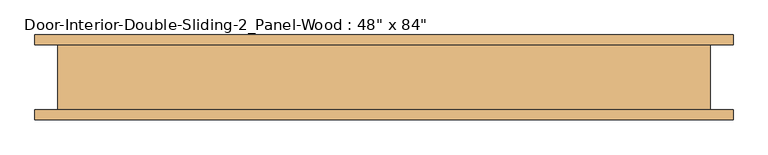
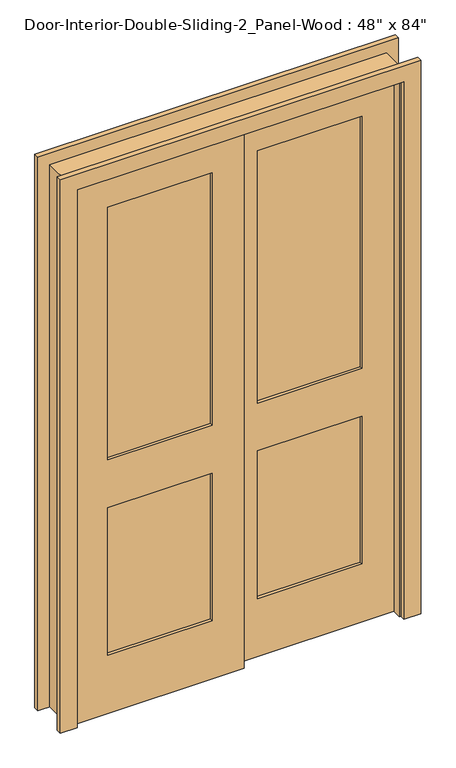
"""IFC4 building model written with IfcOpenShell, lengths in millimetres: door geometry."""

import ifcopenshell
import ifcopenshell.guid

model = None  # the IFC model being written
_history = None  # IfcOwnerHistory: only IFC2X3 demands one
_inside = {}  # id of a spatial element -> (the spatial element, [elements in it])
_under = {}  # id of a project, library or spatial element -> (it, [spatial elements below it])
_declared = {}  # id of a project -> (the project, [libraries it declares])
_typed = {}  # id of a type object -> (the type object, [elements of that type])
_made_of = {}  # id of a material, layer set ... -> (it, [elements and type objects made of it])


def new_model(schema):
    """Start an empty IFC model of exactly this schema.

    Asked for "IFC4X3", IfcOpenShell would pick the latest addendum, in which some entities
    have other attributes; the version numbers below select the first issue.
    IFC2X3 requires an IfcOwnerHistory on every rooted entity: one is made here for all.
    """
    global model, _history
    if schema == "IFC4X3":
        model = ifcopenshell.file(schema_version=(4, 3, 0, 0))
    else:
        model = ifcopenshell.file(schema=schema)
    _inside.clear()
    _under.clear()
    _declared.clear()
    _typed.clear()
    _made_of.clear()
    _history = None
    if model.schema == "IFC2X3":
        org = make("IfcOrganization", Name="unknown")
        user = make(
            "IfcPersonAndOrganization",
            ThePerson=make("IfcPerson", FamilyName="unknown"),
            TheOrganization=org,
        )
        app = make(
            "IfcApplication",
            ApplicationDeveloper=org,
            Version="unknown",
            ApplicationFullName="unknown",
            ApplicationIdentifier="unknown",
        )
        _history = make(
            "IfcOwnerHistory",
            OwningUser=user,
            OwningApplication=app,
            ChangeAction="ADDED",
            CreationDate=0,
        )
    return model


def make(cls, **values):
    """One entity of the class cls with the attributes given. An attribute that is None is left unset."""
    return model.create_entity(
        cls, **{name: value for name, value in values.items() if value is not None}
    )


def rooted(cls, **values):
    """An entity with a GlobalId (a new one), such as an element, a storey or a relation."""
    return make(cls, GlobalId=ifcopenshell.guid.new(), OwnerHistory=_history, **values)


def si_unit(unit_type, name, prefix=None):
    """IfcSIUnit, for example si_unit("LENGTHUNIT", "METRE", prefix="MILLI")."""
    return make("IfcSIUnit", UnitType=unit_type, Prefix=prefix, Name=name)


def assignment(units):
    """IfcUnitAssignment: the units of a project."""
    return None if units is None else make("IfcUnitAssignment", Units=units)


def point(xyz):
    """IfcCartesianPoint."""
    return None if xyz is None else make("IfcCartesianPoint", Coordinates=xyz)


def direction(xyz):
    """IfcDirection."""
    return None if xyz is None else make("IfcDirection", DirectionRatios=xyz)


def frame(location, z_axis=None, x_axis=None):
    """IfcAxis2Placement3D, a coordinate frame: its origin and axes. An axis left out is left unset."""
    return make(
        "IfcAxis2Placement3D",
        Location=point(location),
        Axis=direction(z_axis),
        RefDirection=direction(x_axis),
    )


def origin():
    """The frame at (0, 0, 0) with its axes left unset."""
    return frame((0.0, 0.0, 0.0))


def place(relative_to, where):
    """IfcLocalPlacement: puts the frame where relative to a parent placement (None: the world)."""
    return make(
        "IfcLocalPlacement", PlacementRelTo=relative_to, RelativePlacement=where
    )


def context(
    kind, dimensions, precision=None, world=None, true_north=None, identifier=None
):
    """IfcGeometricRepresentationContext, for example the 3D "Model" context."""
    return make(
        "IfcGeometricRepresentationContext",
        ContextIdentifier=identifier,
        ContextType=kind,
        CoordinateSpaceDimension=dimensions,
        Precision=precision,
        WorldCoordinateSystem=world,
        TrueNorth=true_north,
    )


def project(units=None, contexts=None):
    """IfcProject with its units and contexts."""
    return rooted(
        "IfcProject",
        Name="project",
        RepresentationContexts=contexts,
        UnitsInContext=assignment(units),
    )


def spatial(cls, under=None, at=None, **own):
    """A site, building, storey or space (cls), placed at a placement, below another one or the project."""
    s = rooted(cls, ObjectPlacement=at, **own)
    if under is not None:
        _under.setdefault(under.id(), (under, []))[1].append(s)
    return s


def polyline(points):
    """IfcPolyline through the points."""
    return make("IfcPolyline", Points=[point(p) for p in points])


def outline(outer, holes=None, kind="AREA"):
    """IfcArbitraryClosedProfileDef: a profile drawn as a closed curve; with holes, ...WithVoids."""
    if holes is None:
        return make("IfcArbitraryClosedProfileDef", ProfileType=kind, OuterCurve=outer)
    return make(
        "IfcArbitraryProfileDefWithVoids",
        ProfileType=kind,
        OuterCurve=outer,
        InnerCurves=holes,
    )


def extrude(swept, where, along, depth):
    """IfcExtrudedAreaSolid: the profile swept, set in the frame where, extruded along a direction by depth."""
    return make(
        "IfcExtrudedAreaSolid",
        SweptArea=swept,
        Position=where,
        ExtrudedDirection=direction(along),
        Depth=depth,
    )


def shape(context_of_items, identifier, shape_type, items):
    """IfcShapeRepresentation: the items that make up one representation, for example the "Body"."""
    return make(
        "IfcShapeRepresentation",
        ContextOfItems=context_of_items,
        RepresentationIdentifier=identifier,
        RepresentationType=shape_type,
        Items=items,
    )


def source(mapping_origin, context_of_items, identifier, shape_type, items):
    """IfcRepresentationMap: a shape defined once, which mapped items show again and again."""
    return make(
        "IfcRepresentationMap",
        MappingOrigin=mapping_origin,
        MappedRepresentation=shape(context_of_items, identifier, shape_type, items),
    )


def transform(
    local_origin,
    x_axis=None,
    y_axis=None,
    z_axis=None,
    scale=None,
    scale2=None,
    scale3=None,
    uniform=True,
):
    """IfcCartesianTransformationOperator3D, or its non-uniform kind. x_axis, y_axis, z_axis: its Axis1, 2, 3."""
    if uniform:
        return make(
            "IfcCartesianTransformationOperator3D",
            Axis1=direction(x_axis),
            Axis2=direction(y_axis),
            LocalOrigin=point(local_origin),
            Scale=scale,
            Axis3=direction(z_axis),
        )
    return make(
        "IfcCartesianTransformationOperator3DnonUniform",
        Axis1=direction(x_axis),
        Axis2=direction(y_axis),
        LocalOrigin=point(local_origin),
        Scale=scale,
        Axis3=direction(z_axis),
        Scale2=scale2,
        Scale3=scale3,
    )


def mapped(mapping_source, mapping_target):
    """IfcMappedItem: shows the shape of a source again, moved by a transform."""
    return make(
        "IfcMappedItem", MappingSource=mapping_source, MappingTarget=mapping_target
    )


def made_of(thing, what):
    """Note that an element or type object is made of a material, layer set ...; save() writes the relation."""
    if what is not None:
        _made_of.setdefault(what.id(), (what, []))[1].append(thing)
    return thing


def element(
    cls,
    number,
    at=None,
    inside=None,
    cuts=None,
    type_object=None,
    material=None,
    context=None,
    identifier="Body",
    shape_type=None,
    held_by="IfcProductDefinitionShape",
    body=None,
    shapes=None,
    **own,
):
    """One element of the class cls, such as IfcWall. Its Tag is "e" and its number.

    at: its placement. inside: the storey or other place that contains it. cuts: it is an
    opening in that element (IfcRelVoidsElement). A single representation is given by context,
    identifier, shape_type and body (its items); several are given by shapes. held_by: the class
    of the entity that holds the representations. save() writes the other relations.
    """
    e = rooted(cls, Tag="e%d" % number, ObjectPlacement=at, **own)
    if body is not None:
        shapes = [shape(context, identifier, shape_type, body)]
    if shapes is not None:
        e.Representation = make(held_by, Representations=shapes)
    if inside is not None:
        _inside.setdefault(inside.id(), (inside, []))[1].append(e)
    if cuts is not None:
        rooted(
            "IfcRelVoidsElement", RelatingBuildingElement=cuts, RelatedOpeningElement=e
        )
    if type_object is not None:
        _typed.setdefault(type_object.id(), (type_object, []))[1].append(e)
    return made_of(e, material)


def aggregate(whole, parts):
    """IfcRelAggregates: a whole, such as a stair, and the parts it consists of."""
    return rooted("IfcRelAggregates", RelatingObject=whole, RelatedObjects=parts)


def save(model, path):
    """Write the relations noted so far, then the file.

    IfcRelAggregates (storeys below a building ...), IfcRelContainedInSpatialStructure (elements
    in a storey), IfcRelDefinesByType, IfcRelAssociatesMaterial and IfcRelDeclares: one each for
    every whole, place, type object, material and project.
    """
    for whole, parts in _under.values():
        aggregate(whole, parts)
    for where, things in _inside.values():
        rooted(
            "IfcRelContainedInSpatialStructure",
            RelatedElements=things,
            RelatingStructure=where,
        )
    for kind, things in _typed.values():
        rooted("IfcRelDefinesByType", RelatedObjects=things, RelatingType=kind)
    for what, things in _made_of.values():
        rooted("IfcRelAssociatesMaterial", RelatedObjects=things, RelatingMaterial=what)
    for by, libraries in _declared.values():
        rooted("IfcRelDeclares", RelatingContext=by, RelatedDefinitions=libraries)
    model.write(path)


def door_39e6ccb1(model_context):
    return source(origin(), model_context, "Body", "SweptSolid", [
        extrude(outline(polyline([(488.95, -2.1166667), (488.95, -13.7583333), (95.25, -13.7583333), (95.25, -2.1166667), (488.95, -2.1166667)])), frame((0.0, 0.0, 1009.65), z_axis=(0.0, 0.0, 1.0), x_axis=(1.0, 0.0, 0.0)), (0.0, 0.0, 1.0), 1004.8875),
        extrude(outline(polyline([(488.95, -2.1166667), (488.95, -13.7583333), (95.25, -13.7583333), (95.25, -2.1166667), (488.95, -2.1166667)])), frame((0.0, 0.0, 231.775), z_axis=(0.0, 0.0, 1.0), x_axis=(1.0, 0.0, 0.0)), (0.0, 0.0, 1.0), 587.375),
        extrude(outline(polyline([(2133.6, -25.4), (0.0, -25.4), (0.0, 609.6), (2133.6, 609.6), (2133.6, -25.4)]), holes=[polyline([(2014.5375, 95.25), (2014.5375, 488.95), (1009.65, 488.95), (1009.65, 95.25), (2014.5375, 95.25)]), polyline([(819.15, 95.25), (819.15, 488.95), (231.775, 488.95), (231.775, 95.25), (819.15, 95.25)])]), frame((0.0, -25.4, 0.0), z_axis=(0.0, 1.0, 0.0), x_axis=(0.0, 0.0, 1.0)), (0.0, 0.0, 1.0), 34.925),
        extrude(outline(polyline([(-95.25, -37.0416667), (-95.25, -48.6833333), (-488.95, -48.6833333), (-488.95, -37.0416667), (-95.25, -37.0416667)])), frame((0.0, 0.0, 1009.65), z_axis=(0.0, 0.0, 1.0), x_axis=(1.0, 0.0, 0.0)), (0.0, 0.0, 1.0), 1004.8875),
        extrude(outline(polyline([(-95.25, -37.0416667), (-95.25, -48.6833333), (-488.95, -48.6833333), (-488.95, -37.0416667), (-95.25, -37.0416667)])), frame((0.0, 0.0, 231.775), z_axis=(0.0, 0.0, 1.0), x_axis=(1.0, 0.0, 0.0)), (0.0, 0.0, 1.0), 587.375),
        extrude(outline(polyline([(2133.6, -609.6), (0.0, -609.6), (0.0, 25.4), (2133.6, 25.4), (2133.6, -609.6)]), holes=[polyline([(2014.5375, -488.95), (2014.5375, -95.25), (1009.65, -95.25), (1009.65, -488.95), (2014.5375, -488.95)]), polyline([(819.15, -488.95), (819.15, -95.25), (231.775, -95.25), (231.775, -488.95), (819.15, -488.95)])]), frame((0.0, -60.325, 0.0), z_axis=(0.0, 1.0, 0.0), x_axis=(0.0, 0.0, 1.0)), (0.0, 0.0, 1.0), 34.925),
        extrude(outline(polyline([(0.0, 635.0), (2159.0, 635.0), (2159.0, -635.0), (0.0, -635.0), (0.0, -609.6), (2133.6, -609.6), (2133.6, 609.6), (0.0, 609.6), (0.0, 635.0)])), frame((0.0, -60.325, 0.0), z_axis=(0.0, 1.0, 0.0), x_axis=(0.0, 0.0, 1.0)), (0.0, 0.0, 1.0), 127.0),
        extrude(outline(polyline([(0.0, 679.45), (2203.45, 679.45), (2203.45, -679.45), (0.0, -679.45), (0.0, -615.95), (2139.95, -615.95), (2139.95, 615.95), (0.0, 615.95), (0.0, 679.45)])), frame((0.0, 66.675, 0.0), z_axis=(0.0, 1.0, 0.0), x_axis=(0.0, 0.0, 1.0)), (0.0, 0.0, 1.0), 19.05),
        extrude(outline(polyline([(0.0, 679.45), (2203.45, 679.45), (2203.45, -679.45), (0.0, -679.45), (0.0, -615.95), (2139.95, -615.95), (2139.95, 615.95), (0.0, 615.95), (0.0, 679.45)])), frame((0.0, -79.375, 0.0), z_axis=(0.0, 1.0, 0.0), x_axis=(0.0, 0.0, 1.0)), (0.0, 0.0, 1.0), 19.05),
    ])


if __name__ == "__main__":
    model = new_model("IFC4")
    model_context = context("Model", 3, world=origin())
    ifc_project = project(units=[si_unit("LENGTHUNIT", "METRE", prefix="MILLI")], contexts=[model_context])
    site = spatial("IfcSite", under=ifc_project)
    building = spatial("IfcBuilding", under=site)
    placement = place(None, origin())
    door_shape = door_39e6ccb1(model_context)
    element("IfcDoor", 1, ObjectType="Door-Interior-Double-Sliding-2_Panel-Wood : 48\" x 84\"", at=placement, inside=building, context=model_context, shape_type="MappedRepresentation", body=[
        mapped(door_shape, transform((0.0, 0.0, 0.0), x_axis=(1.0, 0.0, 0.0), y_axis=(0.0, 1.0, 0.0), z_axis=(0.0, 0.0, 1.0))),
    ])
    save(model, "model.ifc")

# Revit data of these elements
# Type "Door-Interior-Double-Sliding-2_Panel-Wood : 48\" x 84\""
#   Type Mark = "13"
#   Assembly Code = "C1020300"
#   Analytic Construction = "Wooden"
#   Top Rail = 0' - 4 11/16"
#   Thickness = 0' - 1 3/8"
#   Thermal Resistance (R) = 2.5876 (h·ft²·°F)/BTU
#   Stiles = 0' - 4 3/4"
#   Rough Width = 4' - 2"
#   Rough Height = 7' - 1"
#   Lock Rail = 0' - 7 1/2"
#   Height = 7' - 0"
#   Width = 4' - 0"
#   Heat Transfer Coefficient (U) = 0.3865 BTU/(h·ft²·°F)
#   Bottom Rail = 0' - 9 1/8"
#   Function = 0
#   Define Thermal Properties by = 1
#   Trim Material = Cherry
#   Panel Material = Cherry
#   Frame Material = Cherry
#   Visual Light Transmittance = 0
#   Solar Heat Gain Coefficient = 0
#   Wall Closure = (empty or 0)
#   Function = (empty or 0)
# Element 1 (IfcDoor, "Door-Interior-Double-Sliding-2_Panel-Wood : 48\" x 84\"")
#   Materials on its faces: "Cherry"
# Materials
#   "Cherry": class "Wood", colour RGB 157 77 38, transparency 0, Description = "Prunus Serotina", Cost = 0
